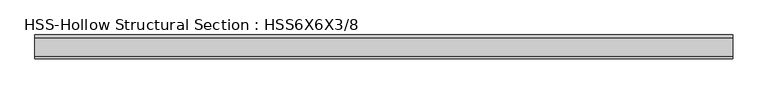
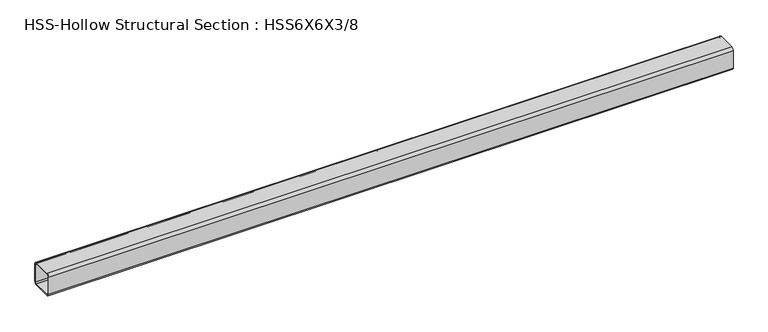
"""IFC4 building model written with IfcOpenShell, lengths in millimetres: member geometry, HSS-Hollow Structural Section : HSS6X6X3/8."""

from ifc_helpers import new_model, si_unit, point, frame, frame_2d, origin, place, context, project, spatial, polyline, circle_curve, trimmed, segment, composite_curve, outline, extrude, source, transform, mapped, element, save


def hss_hollow_structural_section_hss6x6x3_8_6a939be1(model_context):
    return source(origin(), model_context, "Body", "SweptSolid", [
        extrude(outline(composite_curve([segment(polyline([(76.2, 58.4708), (76.2, -58.4708)]), True, "CONTINUOUS"), segment(trimmed(circle_curve(frame_2d((58.4708, -58.4708)), 17.7292), [point((76.2, -58.4708))], [point((58.4708, -76.2))], False, "CARTESIAN"), True, "CONTINUOUS"), segment(polyline([(58.4708, -76.2), (-58.4708, -76.2)]), True, "CONTINUOUS"), segment(trimmed(circle_curve(frame_2d((-58.4708, -58.4708)), 17.7292), [point((-58.4708, -76.2))], [point((-76.2, -58.4708))], False, "CARTESIAN"), True, "CONTINUOUS"), segment(polyline([(-76.2, -58.4708), (-76.2, 58.4708)]), True, "CONTINUOUS"), segment(trimmed(circle_curve(frame_2d((-58.4708, 58.4708)), 17.7292), [point((-76.2, 58.4708))], [point((-58.4708, 76.2))], False, "CARTESIAN"), True, "CONTINUOUS"), segment(polyline([(-58.4708, 76.2), (58.4708, 76.2)]), True, "CONTINUOUS"), segment(trimmed(circle_curve(frame_2d((58.4708, 58.4708)), 17.7292), [point((58.4708, 76.2))], [point((76.2, 58.4708))], False, "CARTESIAN"), True, "CONTINUOUS")], self_intersect=False), holes=[composite_curve([segment(trimmed(circle_curve(frame_2d((-58.4708, 58.4708)), 8.8646), [point((-58.4708, 67.3354))], [point((-67.3354, 58.4708))], True, "CARTESIAN"), True, "CONTINUOUS"), segment(polyline([(-67.3354, 58.4708), (-67.3354, -58.4708)]), True, "CONTINUOUS"), segment(trimmed(circle_curve(frame_2d((-58.4708, -58.4708)), 8.8646), [point((-67.3354, -58.4708))], [point((-58.4708, -67.3354))], True, "CARTESIAN"), True, "CONTINUOUS"), segment(polyline([(-58.4708, -67.3354), (58.4708, -67.3354)]), True, "CONTINUOUS"), segment(trimmed(circle_curve(frame_2d((58.4708, -58.4708)), 8.8646), [point((58.4708, -67.3354))], [point((67.3354, -58.4708))], True, "CARTESIAN"), True, "CONTINUOUS"), segment(polyline([(67.3354, -58.4708), (67.3354, 58.4708)]), True, "CONTINUOUS"), segment(trimmed(circle_curve(frame_2d((58.4708, 58.4708)), 8.8646), [point((67.3354, 58.4708))], [point((58.4708, 67.3354))], True, "CARTESIAN"), True, "CONTINUOUS"), segment(polyline([(58.4708, 67.3354), (-58.4708, 67.3354)]), True, "CONTINUOUS")], self_intersect=False)]), frame((-2205.9552276, 0.0, 0.0), z_axis=(1.0, 0.0, 0.0), x_axis=(0.0, 1.0, 0.0)), (0.0, 0.0, 1.0), 4440.1661943),
    ])


if __name__ == "__main__":
    model = new_model("IFC4")
    model_context = context("Model", 3, world=origin())
    ifc_project = project(units=[si_unit("LENGTHUNIT", "METRE", prefix="MILLI")], contexts=[model_context])
    site = spatial("IfcSite", under=ifc_project)
    building = spatial("IfcBuilding", under=site)
    placement = place(None, origin())
    hss_hollow_structural_section_hss6x6x3_8_shape = hss_hollow_structural_section_hss6x6x3_8_6a939be1(model_context)
    element("IfcMember", 1, ObjectType="HSS-Hollow Structural Section : HSS6X6X3/8", at=placement, inside=building, context=model_context, shape_type="MappedRepresentation", body=[
        mapped(hss_hollow_structural_section_hss6x6x3_8_shape, transform((0.0, 0.0, 0.0), x_axis=(1.0, 0.0, 0.0), y_axis=(0.0, 1.0, 0.0), z_axis=(0.0, 0.0, 1.0))),
    ])
    save(model, "model.ifc")

# Revit data of these elements
# Type "HSS-Hollow Structural Section : HSS6X6X3/8"
#   Assembly Code = "B10"
#   Shape = "Square"
#   W = 27.4
#   Ht = 0' - 6"
#   Length [instance default] = 5' - 0"
#   b = 0' - 6"
#   kr = 0' - 0.698"
#   t = 0' - 0.349"
#   A = 0.0526389 SF
#   Structural Material [instance default] = Steel ASTM A500, Grade B, Rectangular and Square
# Element 1 (IfcMember, "HSS-Hollow Structural Section : HSS6X6X3/8")
#   Materials on its faces: "Steel ASTM A500, Grade B, Rectangular and Square"
# Materials
#   "Steel ASTM A500, Grade B, Rectangular and Square": class "Metal", colour RGB 199 199 199, transparency 0, Description = "Carbon steel", Cost = 0
